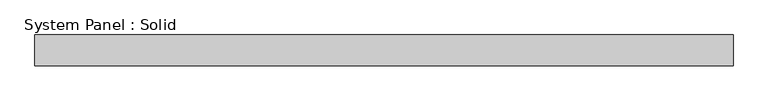
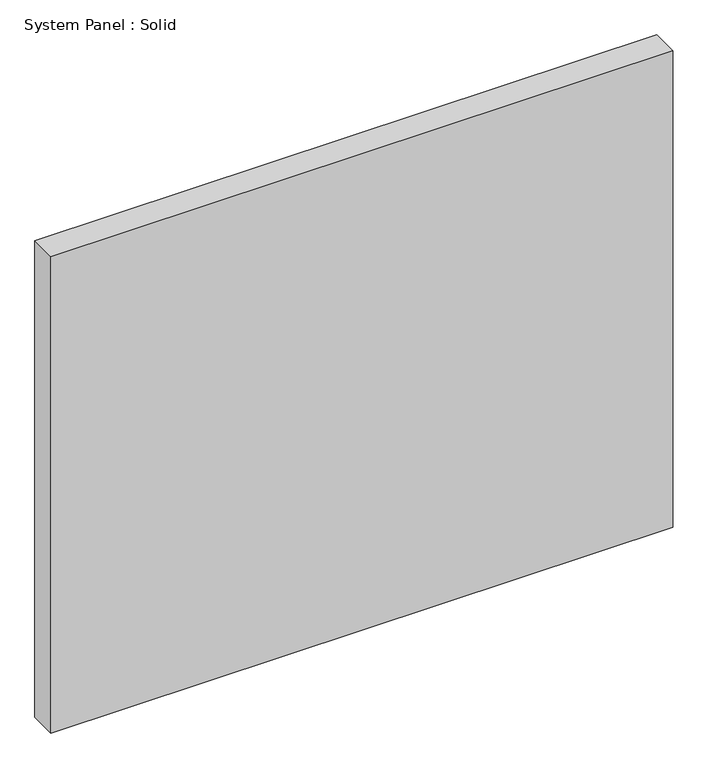
"""IFC4 building model written with IfcOpenShell, lengths in millimetres: plate geometry, System Panel : Solid."""

import ifcopenshell
import ifcopenshell.guid

model = None  # the IFC model being written
_history = None  # IfcOwnerHistory: only IFC2X3 demands one
_inside = {}  # id of a spatial element -> (the spatial element, [elements in it])
_under = {}  # id of a project, library or spatial element -> (it, [spatial elements below it])
_declared = {}  # id of a project -> (the project, [libraries it declares])
_typed = {}  # id of a type object -> (the type object, [elements of that type])
_made_of = {}  # id of a material, layer set ... -> (it, [elements and type objects made of it])


def new_model(schema):
    """Start an empty IFC model of exactly this schema.

    Asked for "IFC4X3", IfcOpenShell would pick the latest addendum, in which some entities
    have other attributes; the version numbers below select the first issue.
    IFC2X3 requires an IfcOwnerHistory on every rooted entity: one is made here for all.
    """
    global model, _history
    if schema == "IFC4X3":
        model = ifcopenshell.file(schema_version=(4, 3, 0, 0))
    else:
        model = ifcopenshell.file(schema=schema)
    _inside.clear()
    _under.clear()
    _declared.clear()
    _typed.clear()
    _made_of.clear()
    _history = None
    if model.schema == "IFC2X3":
        org = make("IfcOrganization", Name="unknown")
        user = make(
            "IfcPersonAndOrganization",
            ThePerson=make("IfcPerson", FamilyName="unknown"),
            TheOrganization=org,
        )
        app = make(
            "IfcApplication",
            ApplicationDeveloper=org,
            Version="unknown",
            ApplicationFullName="unknown",
            ApplicationIdentifier="unknown",
        )
        _history = make(
            "IfcOwnerHistory",
            OwningUser=user,
            OwningApplication=app,
            ChangeAction="ADDED",
            CreationDate=0,
        )
    return model


def make(cls, **values):
    """One entity of the class cls with the attributes given. An attribute that is None is left unset."""
    return model.create_entity(
        cls, **{name: value for name, value in values.items() if value is not None}
    )


def rooted(cls, **values):
    """An entity with a GlobalId (a new one), such as an element, a storey or a relation."""
    return make(cls, GlobalId=ifcopenshell.guid.new(), OwnerHistory=_history, **values)


def si_unit(unit_type, name, prefix=None):
    """IfcSIUnit, for example si_unit("LENGTHUNIT", "METRE", prefix="MILLI")."""
    return make("IfcSIUnit", UnitType=unit_type, Prefix=prefix, Name=name)


def assignment(units):
    """IfcUnitAssignment: the units of a project."""
    return None if units is None else make("IfcUnitAssignment", Units=units)


def point(xyz):
    """IfcCartesianPoint."""
    return None if xyz is None else make("IfcCartesianPoint", Coordinates=xyz)


def direction(xyz):
    """IfcDirection."""
    return None if xyz is None else make("IfcDirection", DirectionRatios=xyz)


def frame(location, z_axis=None, x_axis=None):
    """IfcAxis2Placement3D, a coordinate frame: its origin and axes. An axis left out is left unset."""
    return make(
        "IfcAxis2Placement3D",
        Location=point(location),
        Axis=direction(z_axis),
        RefDirection=direction(x_axis),
    )


def origin():
    """The frame at (0, 0, 0) with its axes left unset."""
    return frame((0.0, 0.0, 0.0))


def origin_with_axes():
    """The frame at (0, 0, 0) with the z axis (0, 0, 1) and the x axis (1, 0, 0) written out."""
    return frame((0.0, 0.0, 0.0), z_axis=(0.0, 0.0, 1.0), x_axis=(1.0, 0.0, 0.0))


def place(relative_to, where):
    """IfcLocalPlacement: puts the frame where relative to a parent placement (None: the world)."""
    return make(
        "IfcLocalPlacement", PlacementRelTo=relative_to, RelativePlacement=where
    )


def context(
    kind, dimensions, precision=None, world=None, true_north=None, identifier=None
):
    """IfcGeometricRepresentationContext, for example the 3D "Model" context."""
    return make(
        "IfcGeometricRepresentationContext",
        ContextIdentifier=identifier,
        ContextType=kind,
        CoordinateSpaceDimension=dimensions,
        Precision=precision,
        WorldCoordinateSystem=world,
        TrueNorth=true_north,
    )


def project(units=None, contexts=None):
    """IfcProject with its units and contexts."""
    return rooted(
        "IfcProject",
        Name="project",
        RepresentationContexts=contexts,
        UnitsInContext=assignment(units),
    )


def spatial(cls, under=None, at=None, **own):
    """A site, building, storey or space (cls), placed at a placement, below another one or the project."""
    s = rooted(cls, ObjectPlacement=at, **own)
    if under is not None:
        _under.setdefault(under.id(), (under, []))[1].append(s)
    return s


def polyline(points):
    """IfcPolyline through the points."""
    return make("IfcPolyline", Points=[point(p) for p in points])


def outline(outer, holes=None, kind="AREA"):
    """IfcArbitraryClosedProfileDef: a profile drawn as a closed curve; with holes, ...WithVoids."""
    if holes is None:
        return make("IfcArbitraryClosedProfileDef", ProfileType=kind, OuterCurve=outer)
    return make(
        "IfcArbitraryProfileDefWithVoids",
        ProfileType=kind,
        OuterCurve=outer,
        InnerCurves=holes,
    )


def extrude(swept, where, along, depth):
    """IfcExtrudedAreaSolid: the profile swept, set in the frame where, extruded along a direction by depth."""
    return make(
        "IfcExtrudedAreaSolid",
        SweptArea=swept,
        Position=where,
        ExtrudedDirection=direction(along),
        Depth=depth,
    )


def shape(context_of_items, identifier, shape_type, items):
    """IfcShapeRepresentation: the items that make up one representation, for example the "Body"."""
    return make(
        "IfcShapeRepresentation",
        ContextOfItems=context_of_items,
        RepresentationIdentifier=identifier,
        RepresentationType=shape_type,
        Items=items,
    )


def source(mapping_origin, context_of_items, identifier, shape_type, items):
    """IfcRepresentationMap: a shape defined once, which mapped items show again and again."""
    return make(
        "IfcRepresentationMap",
        MappingOrigin=mapping_origin,
        MappedRepresentation=shape(context_of_items, identifier, shape_type, items),
    )


def transform(
    local_origin,
    x_axis=None,
    y_axis=None,
    z_axis=None,
    scale=None,
    scale2=None,
    scale3=None,
    uniform=True,
):
    """IfcCartesianTransformationOperator3D, or its non-uniform kind. x_axis, y_axis, z_axis: its Axis1, 2, 3."""
    if uniform:
        return make(
            "IfcCartesianTransformationOperator3D",
            Axis1=direction(x_axis),
            Axis2=direction(y_axis),
            LocalOrigin=point(local_origin),
            Scale=scale,
            Axis3=direction(z_axis),
        )
    return make(
        "IfcCartesianTransformationOperator3DnonUniform",
        Axis1=direction(x_axis),
        Axis2=direction(y_axis),
        LocalOrigin=point(local_origin),
        Scale=scale,
        Axis3=direction(z_axis),
        Scale2=scale2,
        Scale3=scale3,
    )


def mapped(mapping_source, mapping_target):
    """IfcMappedItem: shows the shape of a source again, moved by a transform."""
    return make(
        "IfcMappedItem", MappingSource=mapping_source, MappingTarget=mapping_target
    )


def made_of(thing, what):
    """Note that an element or type object is made of a material, layer set ...; save() writes the relation."""
    if what is not None:
        _made_of.setdefault(what.id(), (what, []))[1].append(thing)
    return thing


def element(
    cls,
    number,
    at=None,
    inside=None,
    cuts=None,
    type_object=None,
    material=None,
    context=None,
    identifier="Body",
    shape_type=None,
    held_by="IfcProductDefinitionShape",
    body=None,
    shapes=None,
    **own,
):
    """One element of the class cls, such as IfcWall. Its Tag is "e" and its number.

    at: its placement. inside: the storey or other place that contains it. cuts: it is an
    opening in that element (IfcRelVoidsElement). A single representation is given by context,
    identifier, shape_type and body (its items); several are given by shapes. held_by: the class
    of the entity that holds the representations. save() writes the other relations.
    """
    e = rooted(cls, Tag="e%d" % number, ObjectPlacement=at, **own)
    if body is not None:
        shapes = [shape(context, identifier, shape_type, body)]
    if shapes is not None:
        e.Representation = make(held_by, Representations=shapes)
    if inside is not None:
        _inside.setdefault(inside.id(), (inside, []))[1].append(e)
    if cuts is not None:
        rooted(
            "IfcRelVoidsElement", RelatingBuildingElement=cuts, RelatedOpeningElement=e
        )
    if type_object is not None:
        _typed.setdefault(type_object.id(), (type_object, []))[1].append(e)
    return made_of(e, material)


def aggregate(whole, parts):
    """IfcRelAggregates: a whole, such as a stair, and the parts it consists of."""
    return rooted("IfcRelAggregates", RelatingObject=whole, RelatedObjects=parts)


def save(model, path):
    """Write the relations noted so far, then the file.

    IfcRelAggregates (storeys below a building ...), IfcRelContainedInSpatialStructure (elements
    in a storey), IfcRelDefinesByType, IfcRelAssociatesMaterial and IfcRelDeclares: one each for
    every whole, place, type object, material and project.
    """
    for whole, parts in _under.values():
        aggregate(whole, parts)
    for where, things in _inside.values():
        rooted(
            "IfcRelContainedInSpatialStructure",
            RelatedElements=things,
            RelatingStructure=where,
        )
    for kind, things in _typed.values():
        rooted("IfcRelDefinesByType", RelatedObjects=things, RelatingType=kind)
    for what, things in _made_of.values():
        rooted("IfcRelAssociatesMaterial", RelatedObjects=things, RelatingMaterial=what)
    for by, libraries in _declared.values():
        rooted("IfcRelDeclares", RelatingContext=by, RelatedDefinitions=libraries)
    model.write(path)


def system_panel_solid_db88bede(model_context):
    return source(origin(), model_context, "Body", "SweptSolid", [
        extrude(outline(polyline([(713.3166666, -44.45), (-713.3166666, -44.45), (-713.3166666, 19.05), (713.3166666, 19.05), (713.3166666, -44.45)])), origin_with_axes(), (0.0, 0.0, 1.0), 1155.7),
    ])


if __name__ == "__main__":
    model = new_model("IFC4")
    model_context = context("Model", 3, world=origin())
    ifc_project = project(units=[si_unit("LENGTHUNIT", "METRE", prefix="MILLI")], contexts=[model_context])
    site = spatial("IfcSite", under=ifc_project)
    building = spatial("IfcBuilding", under=site)
    placement = place(None, origin())
    system_panel_solid_shape = system_panel_solid_db88bede(model_context)
    element("IfcPlate", 1, ObjectType="System Panel : Solid", at=placement, inside=building, context=model_context, shape_type="MappedRepresentation", body=[
        mapped(system_panel_solid_shape, transform((0.0, 0.0, 0.0), x_axis=(1.0, 0.0, 0.0), y_axis=(0.0, 1.0, 0.0), z_axis=(0.0, 0.0, 1.0))),
    ])
    save(model, "model.ifc")

# Revit data of these elements
# Type "System Panel : Solid"
#   Construction Type Id = "MDOOR"
#   Analytic Construction = "Metal"
#   Visual Light Transmittance = 0
#   Solar Heat Gain Coefficient = 0
#   Heat Transfer Coefficient (U) = 0.651978 BTU/(h·ft²·°F)
#   Define Thermal Properties by = 1
# Element 1 (IfcPlate, "System Panel : Solid")
#   Materials on its faces: "Default"
# Materials
#   "Default": class "Miscellaneous", colour RGB 127 127 127, transparency 0, Cost = 0
